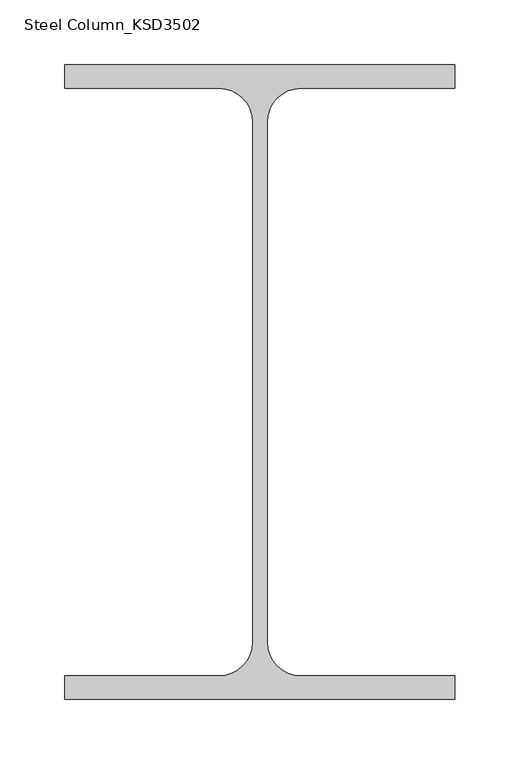
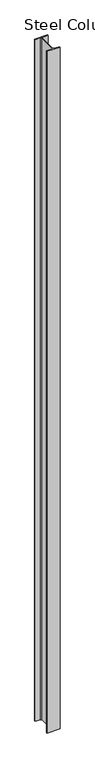
"""IFC4 building model written with IfcOpenShell, lengths in millimetres: column geometry, Steel Column_KSD3502 : H_SC_ASC_H-488×300x11x18."""

from ifc_helpers import new_model, si_unit, point, frame, frame_2d, origin, place, context, project, spatial, polyline, circle_curve, trimmed, segment, composite_curve, outline, extrude, source, transform, mapped, element, save


def steel_column_ksd3502_8b02a347(model_context):
    return source(origin(), model_context, "Body", "SweptSolid", [
        extrude(outline(composite_curve([segment(polyline([(150.0, 244.0), (150.0, 226.0), (31.5, 226.0)]), True, "CONTINUOUS"), segment(trimmed(circle_curve(frame_2d((31.5, 200.0)), 26.0), [point((31.5, 226.0))], [point((5.5, 200.0))], True, "CARTESIAN"), True, "CONTINUOUS"), segment(polyline([(5.5, 200.0), (5.5, -200.0)]), True, "CONTINUOUS"), segment(trimmed(circle_curve(frame_2d((31.5, -200.0)), 26.0), [point((5.5, -200.0))], [point((31.5, -226.0))], True, "CARTESIAN"), True, "CONTINUOUS"), segment(polyline([(31.5, -226.0), (150.0, -226.0), (150.0, -244.0), (-150.0, -244.0), (-150.0, -226.0), (-31.5, -226.0)]), True, "CONTINUOUS"), segment(trimmed(circle_curve(frame_2d((-31.5, -200.0)), 26.0), [point((-31.5, -226.0))], [point((-5.5, -200.0))], True, "CARTESIAN"), True, "CONTINUOUS"), segment(polyline([(-5.5, -200.0), (-5.5, 200.0)]), True, "CONTINUOUS"), segment(trimmed(circle_curve(frame_2d((-31.5, 200.0)), 26.0), [point((-5.5, 200.0))], [point((-31.5, 226.0))], True, "CARTESIAN"), True, "CONTINUOUS"), segment(polyline([(-31.5, 226.0), (-150.0, 226.0), (-150.0, 244.0), (150.0, 244.0)]), True, "CONTINUOUS")], self_intersect=False)), frame((0.0, 0.0, 685.9720055), z_axis=(0.0, 0.0, 1.0), x_axis=(1.0, 0.0, 0.0)), (0.0, 0.0, 1.0), 16614.0),
    ])


if __name__ == "__main__":
    model = new_model("IFC4")
    model_context = context("Model", 3, world=origin())
    ifc_project = project(units=[si_unit("LENGTHUNIT", "METRE", prefix="MILLI")], contexts=[model_context])
    site = spatial("IfcSite", under=ifc_project)
    building = spatial("IfcBuilding", under=site)
    placement = place(None, origin())
    steel_column_ksd3502_shape = steel_column_ksd3502_8b02a347(model_context)
    element("IfcColumn", 1, ObjectType="Steel Column_KSD3502 : H_SC_ASC_H-488×300x11x18", at=placement, inside=building, context=model_context, shape_type="MappedRepresentation", body=[
        mapped(steel_column_ksd3502_shape, transform((0.0, 0.0, 0.0), x_axis=(1.0, 0.0, 0.0), y_axis=(0.0, 1.0, 0.0), z_axis=(0.0, 0.0, 1.0))),
    ])
    save(model, "model.ifc")

# Revit data of these elements
# Type "Steel Column_KSD3502 : H_SC_ASC_H-488×300x11x18"
#   Width = 30.0 cm
#   Web Thickness = 1.1 cm
#   Web Fillet = 2.6 cm
#   Warping Constant = 4473230.0 cm⁶
#   Torsional Moment of Inertia = 137.492 cm⁴
#   Section Area = 163.5 cm²
#   Plastic Modulus weak axis = 830.0 cm³
#   Plastic Modulus strong axis = 3230.0 cm³
#   Perimeter = 1.27 m²/m
#   Nominal Weight = 128.00 kgf/m
#   Moment of Inertia weak axis = 8110.00 cm⁴
#   Moment of Inertia strong axis = 71000.00 cm⁴
#   Height = 48.8 cm
#   Flange Thickness = 1.8 cm
#   Elastic Modulus weak axis = 541.0 cm³
#   Elastic Modulus strong axis = 2910.0 cm³
#   Centroid Vertical = 24.4 cm
#   Centroid Horizontal = 15.0 cm
#   Bolt Spacing = 13.97 cm
#   Structural Material [instance default] = Steel, 45-345
#   Section Name Key = ""
#   Assembly Code = ""
# Element 1 (IfcColumn, "Steel Column_KSD3502 : H_SC_ASC_H-488×300x11x18")
#   Structural Material = A03AD029-00005_Anchor Bolt (Installation only)_M24
#   Materials on its faces: "A03AD029-00005_Anchor Bolt (Installation only)_M24"
# Materials
#   "Steel, 45-345": class "Metal", colour RGB 189 187 185, transparency 0, Description = "Steel 345 MPa", Cost = 0
#   "A03AD029-00005_Anchor Bolt (Installation only)_M24": class "Unassigned", colour RGB 84 83 81, transparency 0, Cost = 0
